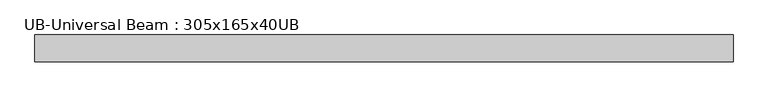
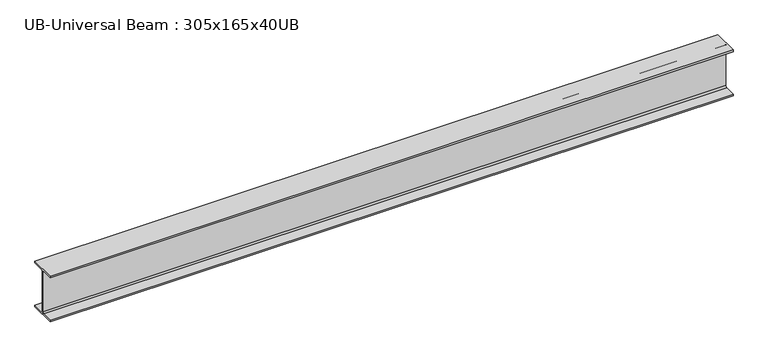
"""IFC4 building model written with IfcOpenShell, lengths in millimetres: beam geometry, UB-Universal Beam : 305x165x40UB."""

from ifc_helpers import new_model, si_unit, point, frame, frame_2d, origin, place, context, project, spatial, polyline, circle_curve, trimmed, segment, composite_curve, outline, extrude, source, transform, mapped, element, save


def ub_universal_beam_305x165x40ub_980d3c35(model_context):
    return source(origin(), model_context, "Body", "SweptSolid", [
        extrude(outline(composite_curve([segment(polyline([(82.5, -141.5), (82.5, -151.7), (-82.5, -151.7), (-82.5, -141.5), (-11.9, -141.5)]), True, "CONTINUOUS"), segment(trimmed(circle_curve(frame_2d((-11.9, -132.6)), 8.9), [point((-11.9, -141.5))], [point((-3.0, -132.6))], True, "CARTESIAN"), True, "CONTINUOUS"), segment(polyline([(-3.0, -132.6), (-3.0, 132.6)]), True, "CONTINUOUS"), segment(trimmed(circle_curve(frame_2d((-11.9, 132.6)), 8.9), [point((-3.0, 132.6))], [point((-11.9, 141.5))], True, "CARTESIAN"), True, "CONTINUOUS"), segment(polyline([(-11.9, 141.5), (-82.5, 141.5), (-82.5, 151.7), (82.5, 151.7), (82.5, 141.5), (11.9, 141.5)]), True, "CONTINUOUS"), segment(trimmed(circle_curve(frame_2d((11.9, 132.6)), 8.9), [point((11.9, 141.5))], [point((3.0, 132.6))], True, "CARTESIAN"), True, "CONTINUOUS"), segment(polyline([(3.0, 132.6), (3.0, -132.6)]), True, "CONTINUOUS"), segment(trimmed(circle_curve(frame_2d((11.9, -132.6)), 8.9), [point((3.0, -132.6))], [point((11.9, -141.5))], True, "CARTESIAN"), True, "CONTINUOUS"), segment(polyline([(11.9, -141.5), (82.5, -141.5)]), True, "CONTINUOUS")], self_intersect=False)), frame((-2134.65, 0.0, 0.0), z_axis=(1.0, 0.0, 0.0), x_axis=(0.0, 1.0, 0.0)), (0.0, 0.0, 1.0), 4293.0),
    ])


if __name__ == "__main__":
    model = new_model("IFC4")
    model_context = context("Model", 3, world=origin())
    ifc_project = project(units=[si_unit("LENGTHUNIT", "METRE", prefix="MILLI")], contexts=[model_context])
    site = spatial("IfcSite", under=ifc_project)
    building = spatial("IfcBuilding", under=site)
    placement = place(None, origin())
    ub_universal_beam_305x165x40ub_shape = ub_universal_beam_305x165x40ub_980d3c35(model_context)
    element("IfcBeam", 1, ObjectType="UB-Universal Beam : 305x165x40UB", at=placement, inside=building, context=model_context, shape_type="MappedRepresentation", body=[
        mapped(ub_universal_beam_305x165x40ub_shape, transform((0.0, 0.0, 0.0), x_axis=(1.0, 0.0, 0.0), y_axis=(0.0, 1.0, 0.0), z_axis=(0.0, 0.0, 1.0))),
    ])
    save(model, "model.ifc")

# Revit data of these elements
# Type "UB-Universal Beam : 305x165x40UB"
#   Nominal h = "305"
#   W = 0
#   Start Extension Calculation [instance default] = 3000 mm
#   Start Extension [instance default] = -12.7 mm
#   End Extension Calculation [instance default] = 3000 mm
#   End Extension [instance default] = -12.7 mm
#   Ix = 8503
#   Length [instance default] = 1524 mm
#   M = 40.3
#   Zx = 560
#   b = 165 mm
#   h = 303.4 mm
#   r = 8.9 mm
#   s = 6 mm
#   t = 10.2 mm
#   A = 0.005 m²
#   Structural Material [instance default] = Metal - Steel - 345 MPa
#   Assembly Code = ""
# Element 1 (IfcBeam, "UB-Universal Beam : 305x165x40UB")
#   Materials on its faces: "Metal - Steel - 345 MPa"
# Materials
#   "Metal - Steel - 345 MPa": class "Metal", colour RGB 241 46 46, transparency 0
